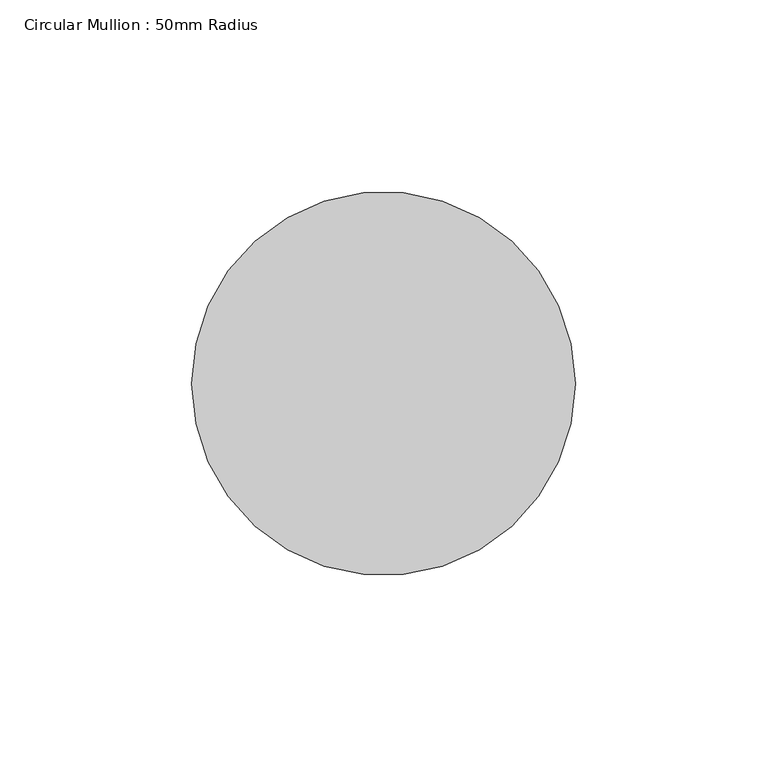
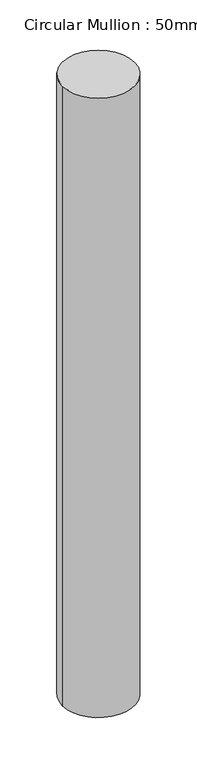
"""IFC4 building model written with IfcOpenShell, lengths in millimetres: member geometry, Circular Mullion : 50mm Radius."""

import ifcopenshell
import ifcopenshell.guid

model = None  # the IFC model being written
_history = None  # IfcOwnerHistory: only IFC2X3 demands one
_inside = {}  # id of a spatial element -> (the spatial element, [elements in it])
_under = {}  # id of a project, library or spatial element -> (it, [spatial elements below it])
_declared = {}  # id of a project -> (the project, [libraries it declares])
_typed = {}  # id of a type object -> (the type object, [elements of that type])
_made_of = {}  # id of a material, layer set ... -> (it, [elements and type objects made of it])


def new_model(schema):
    """Start an empty IFC model of exactly this schema.

    Asked for "IFC4X3", IfcOpenShell would pick the latest addendum, in which some entities
    have other attributes; the version numbers below select the first issue.
    IFC2X3 requires an IfcOwnerHistory on every rooted entity: one is made here for all.
    """
    global model, _history
    if schema == "IFC4X3":
        model = ifcopenshell.file(schema_version=(4, 3, 0, 0))
    else:
        model = ifcopenshell.file(schema=schema)
    _inside.clear()
    _under.clear()
    _declared.clear()
    _typed.clear()
    _made_of.clear()
    _history = None
    if model.schema == "IFC2X3":
        org = make("IfcOrganization", Name="unknown")
        user = make(
            "IfcPersonAndOrganization",
            ThePerson=make("IfcPerson", FamilyName="unknown"),
            TheOrganization=org,
        )
        app = make(
            "IfcApplication",
            ApplicationDeveloper=org,
            Version="unknown",
            ApplicationFullName="unknown",
            ApplicationIdentifier="unknown",
        )
        _history = make(
            "IfcOwnerHistory",
            OwningUser=user,
            OwningApplication=app,
            ChangeAction="ADDED",
            CreationDate=0,
        )
    return model


def make(cls, **values):
    """One entity of the class cls with the attributes given. An attribute that is None is left unset."""
    return model.create_entity(
        cls, **{name: value for name, value in values.items() if value is not None}
    )


def rooted(cls, **values):
    """An entity with a GlobalId (a new one), such as an element, a storey or a relation."""
    return make(cls, GlobalId=ifcopenshell.guid.new(), OwnerHistory=_history, **values)


def si_unit(unit_type, name, prefix=None):
    """IfcSIUnit, for example si_unit("LENGTHUNIT", "METRE", prefix="MILLI")."""
    return make("IfcSIUnit", UnitType=unit_type, Prefix=prefix, Name=name)


def assignment(units):
    """IfcUnitAssignment: the units of a project."""
    return None if units is None else make("IfcUnitAssignment", Units=units)


def point(xyz):
    """IfcCartesianPoint."""
    return None if xyz is None else make("IfcCartesianPoint", Coordinates=xyz)


def direction(xyz):
    """IfcDirection."""
    return None if xyz is None else make("IfcDirection", DirectionRatios=xyz)


def frame(location, z_axis=None, x_axis=None):
    """IfcAxis2Placement3D, a coordinate frame: its origin and axes. An axis left out is left unset."""
    return make(
        "IfcAxis2Placement3D",
        Location=point(location),
        Axis=direction(z_axis),
        RefDirection=direction(x_axis),
    )


def frame_2d(location, x_axis=None):
    """IfcAxis2Placement2D, a coordinate frame in the plane: its origin and x axis."""
    return make(
        "IfcAxis2Placement2D", Location=point(location), RefDirection=direction(x_axis)
    )


def origin():
    """The frame at (0, 0, 0) with its axes left unset."""
    return frame((0.0, 0.0, 0.0))


def origin_2d():
    """The frame at (0, 0) in the plane with its x axis left unset."""
    return frame_2d((0.0, 0.0))


def place(relative_to, where):
    """IfcLocalPlacement: puts the frame where relative to a parent placement (None: the world)."""
    return make(
        "IfcLocalPlacement", PlacementRelTo=relative_to, RelativePlacement=where
    )


def context(
    kind, dimensions, precision=None, world=None, true_north=None, identifier=None
):
    """IfcGeometricRepresentationContext, for example the 3D "Model" context."""
    return make(
        "IfcGeometricRepresentationContext",
        ContextIdentifier=identifier,
        ContextType=kind,
        CoordinateSpaceDimension=dimensions,
        Precision=precision,
        WorldCoordinateSystem=world,
        TrueNorth=true_north,
    )


def project(units=None, contexts=None):
    """IfcProject with its units and contexts."""
    return rooted(
        "IfcProject",
        Name="project",
        RepresentationContexts=contexts,
        UnitsInContext=assignment(units),
    )


def spatial(cls, under=None, at=None, **own):
    """A site, building, storey or space (cls), placed at a placement, below another one or the project."""
    s = rooted(cls, ObjectPlacement=at, **own)
    if under is not None:
        _under.setdefault(under.id(), (under, []))[1].append(s)
    return s


def circle_curve(where, radius):
    """IfcCircle in the frame where."""
    return make("IfcCircle", Position=where, Radius=radius)


def trimmed(basis, trim1, trim2, sense, master):
    """IfcTrimmedCurve: the piece of a basis curve between two trims."""
    return make(
        "IfcTrimmedCurve",
        BasisCurve=basis,
        Trim1=trim1,
        Trim2=trim2,
        SenseAgreement=sense,
        MasterRepresentation=master,
    )


def segment(curve, same_sense, transition):
    """IfcCompositeCurveSegment."""
    return make(
        "IfcCompositeCurveSegment",
        Transition=transition,
        SameSense=same_sense,
        ParentCurve=curve,
    )


def composite_curve(segments, self_intersect=None):
    """IfcCompositeCurve: segments joined end to end."""
    return make("IfcCompositeCurve", Segments=segments, SelfIntersect=self_intersect)


def outline(outer, holes=None, kind="AREA"):
    """IfcArbitraryClosedProfileDef: a profile drawn as a closed curve; with holes, ...WithVoids."""
    if holes is None:
        return make("IfcArbitraryClosedProfileDef", ProfileType=kind, OuterCurve=outer)
    return make(
        "IfcArbitraryProfileDefWithVoids",
        ProfileType=kind,
        OuterCurve=outer,
        InnerCurves=holes,
    )


def extrude(swept, where, along, depth):
    """IfcExtrudedAreaSolid: the profile swept, set in the frame where, extruded along a direction by depth."""
    return make(
        "IfcExtrudedAreaSolid",
        SweptArea=swept,
        Position=where,
        ExtrudedDirection=direction(along),
        Depth=depth,
    )


def shape(context_of_items, identifier, shape_type, items):
    """IfcShapeRepresentation: the items that make up one representation, for example the "Body"."""
    return make(
        "IfcShapeRepresentation",
        ContextOfItems=context_of_items,
        RepresentationIdentifier=identifier,
        RepresentationType=shape_type,
        Items=items,
    )


def source(mapping_origin, context_of_items, identifier, shape_type, items):
    """IfcRepresentationMap: a shape defined once, which mapped items show again and again."""
    return make(
        "IfcRepresentationMap",
        MappingOrigin=mapping_origin,
        MappedRepresentation=shape(context_of_items, identifier, shape_type, items),
    )


def transform(
    local_origin,
    x_axis=None,
    y_axis=None,
    z_axis=None,
    scale=None,
    scale2=None,
    scale3=None,
    uniform=True,
):
    """IfcCartesianTransformationOperator3D, or its non-uniform kind. x_axis, y_axis, z_axis: its Axis1, 2, 3."""
    if uniform:
        return make(
            "IfcCartesianTransformationOperator3D",
            Axis1=direction(x_axis),
            Axis2=direction(y_axis),
            LocalOrigin=point(local_origin),
            Scale=scale,
            Axis3=direction(z_axis),
        )
    return make(
        "IfcCartesianTransformationOperator3DnonUniform",
        Axis1=direction(x_axis),
        Axis2=direction(y_axis),
        LocalOrigin=point(local_origin),
        Scale=scale,
        Axis3=direction(z_axis),
        Scale2=scale2,
        Scale3=scale3,
    )


def mapped(mapping_source, mapping_target):
    """IfcMappedItem: shows the shape of a source again, moved by a transform."""
    return make(
        "IfcMappedItem", MappingSource=mapping_source, MappingTarget=mapping_target
    )


def made_of(thing, what):
    """Note that an element or type object is made of a material, layer set ...; save() writes the relation."""
    if what is not None:
        _made_of.setdefault(what.id(), (what, []))[1].append(thing)
    return thing


def element(
    cls,
    number,
    at=None,
    inside=None,
    cuts=None,
    type_object=None,
    material=None,
    context=None,
    identifier="Body",
    shape_type=None,
    held_by="IfcProductDefinitionShape",
    body=None,
    shapes=None,
    **own,
):
    """One element of the class cls, such as IfcWall. Its Tag is "e" and its number.

    at: its placement. inside: the storey or other place that contains it. cuts: it is an
    opening in that element (IfcRelVoidsElement). A single representation is given by context,
    identifier, shape_type and body (its items); several are given by shapes. held_by: the class
    of the entity that holds the representations. save() writes the other relations.
    """
    e = rooted(cls, Tag="e%d" % number, ObjectPlacement=at, **own)
    if body is not None:
        shapes = [shape(context, identifier, shape_type, body)]
    if shapes is not None:
        e.Representation = make(held_by, Representations=shapes)
    if inside is not None:
        _inside.setdefault(inside.id(), (inside, []))[1].append(e)
    if cuts is not None:
        rooted(
            "IfcRelVoidsElement", RelatingBuildingElement=cuts, RelatedOpeningElement=e
        )
    if type_object is not None:
        _typed.setdefault(type_object.id(), (type_object, []))[1].append(e)
    return made_of(e, material)


def aggregate(whole, parts):
    """IfcRelAggregates: a whole, such as a stair, and the parts it consists of."""
    return rooted("IfcRelAggregates", RelatingObject=whole, RelatedObjects=parts)


def save(model, path):
    """Write the relations noted so far, then the file.

    IfcRelAggregates (storeys below a building ...), IfcRelContainedInSpatialStructure (elements
    in a storey), IfcRelDefinesByType, IfcRelAssociatesMaterial and IfcRelDeclares: one each for
    every whole, place, type object, material and project.
    """
    for whole, parts in _under.values():
        aggregate(whole, parts)
    for where, things in _inside.values():
        rooted(
            "IfcRelContainedInSpatialStructure",
            RelatedElements=things,
            RelatingStructure=where,
        )
    for kind, things in _typed.values():
        rooted("IfcRelDefinesByType", RelatedObjects=things, RelatingType=kind)
    for what, things in _made_of.values():
        rooted("IfcRelAssociatesMaterial", RelatedObjects=things, RelatingMaterial=what)
    for by, libraries in _declared.values():
        rooted("IfcRelDeclares", RelatingContext=by, RelatedDefinitions=libraries)
    model.write(path)


def circular_mullion_50mm_radius_033f0597(model_context):
    return source(origin(), model_context, "Body", "SweptSolid", [
        extrude(outline(composite_curve([segment(trimmed(circle_curve(origin_2d(), 50.0), [point((50.0, 0.0))], [point((-50.0, 0.0))], False, "CARTESIAN"), True, "CONTINUOUS"), segment(trimmed(circle_curve(origin_2d(), 50.0), [point((-50.0, 0.0))], [point((50.0, 0.0))], False, "CARTESIAN"), True, "CONTINUOUS")], self_intersect=False)), frame((0.0, 0.0, -908.9514653), z_axis=(0.0, 0.0, 1.0), x_axis=(1.0, 0.0, 0.0)), (0.0, 0.0, 1.0), 908.9514653),
    ])


if __name__ == "__main__":
    model = new_model("IFC4")
    model_context = context("Model", 3, world=origin())
    ifc_project = project(units=[si_unit("LENGTHUNIT", "METRE", prefix="MILLI")], contexts=[model_context])
    site = spatial("IfcSite", under=ifc_project)
    building = spatial("IfcBuilding", under=site)
    placement = place(None, origin())
    circular_mullion_50mm_radius_shape = circular_mullion_50mm_radius_033f0597(model_context)
    element("IfcMember", 1, ObjectType="Circular Mullion : 50mm Radius", at=placement, inside=building, context=model_context, shape_type="MappedRepresentation", body=[
        mapped(circular_mullion_50mm_radius_shape, transform((0.0, 0.0, 0.0), x_axis=(1.0, 0.0, 0.0), y_axis=(0.0, 1.0, 0.0), z_axis=(0.0, 0.0, 1.0))),
    ])
    save(model, "model.ifc")

# Revit data of these elements
# Type "Circular Mullion : 50mm Radius"
#   built-in parameter 1007350 = 0.164042 (stored number, unit not read)
# Element 1 (IfcMember, "Circular Mullion : 50mm Radius")
#   Materials on its faces: "Aluminium"
# Materials
#   "Aluminium": class "Metal", colour RGB 247 247 247, transparency 0, Description = "Aluminium 6061", Cost = 0
